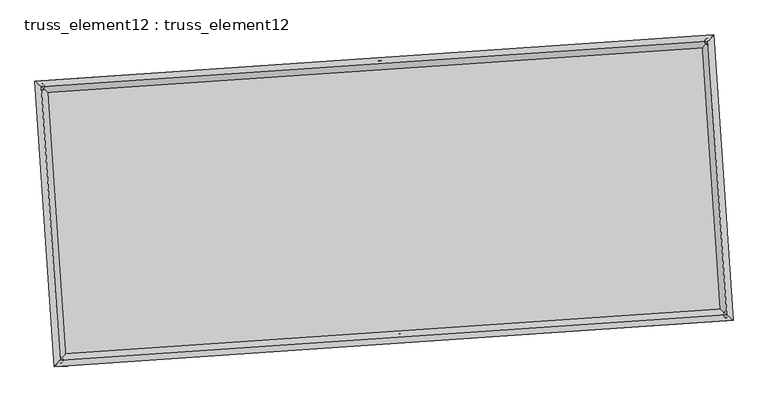
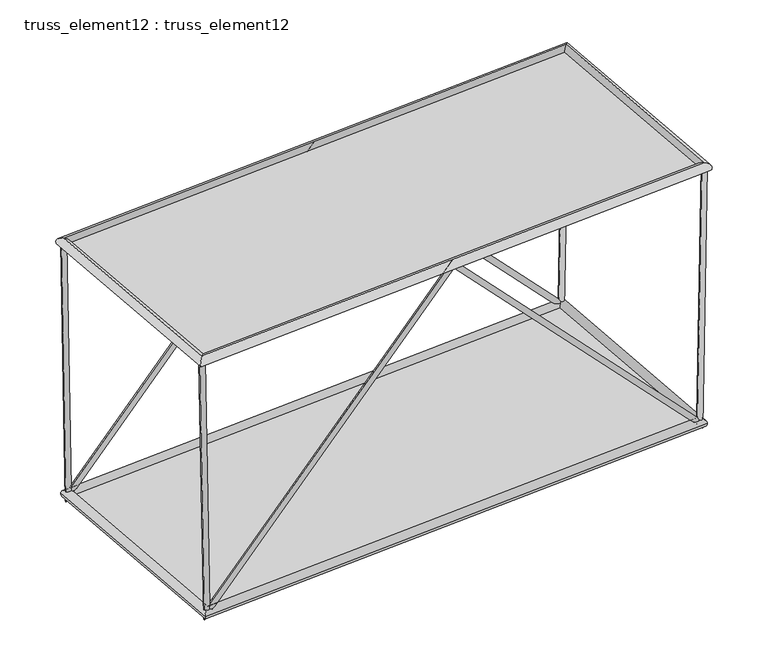
"""IFC4 building model written with IfcOpenShell, lengths in millimetres: plate geometry, truss_element12 : truss_element12."""

from ifc_helpers import new_model, si_unit, frame, origin, origin_with_axes, place, context, project, spatial, polyline, circle_curve, ellipse_curve, outline, extrude, source, transform, mapped, element, save
from ifc_brep_helpers import plane_surface, cylinder_surface, advanced_brep


def truss_element12_truss_element12_2665aa7a(model_context):
    return source(origin(), model_context, "Body", "SolidModel", [
        advanced_brep(
        [(-3754.7580634, 2270.0997186, 5000.0878443), (-3853.8452977, 2256.7395966, 4998.2914205), (-3667.1235212, 2276.0751849, 121.8973883), (-3761.8633617, 2263.0114952, -121.8973883), (1064.4357247, 2598.7022236, 5071.2944643), (1064.8732295, 2592.1283152, 4927.0589346), (5794.5966137, 2921.2339136, 121.8875614), (5890.1643633, 2921.1465749, -121.8875614), (5883.6190751, 2927.3040168, 5000.0761995), (5983.6021946, 2927.5177455, 4998.2513335)],
        [
            (0, 1, circle_curve(frame((-3804.3016806, 2263.4196576, 4999.1896324), z_axis=(-0.01796164783284105, -0.001224736487108711, 0.9998379264799201), x_axis=(-0.13360156854289684, 0.9910344161296608, -0.0011861405566435394)), 50.0)),
            (1, 0, circle_curve(frame((-3804.3016806, 2263.4196576, 4999.1896324), z_axis=(-0.01796164783284105, -0.001224736487108711, 0.9998379264799201), x_axis=(-0.13360156854289684, 0.9910344161296608, -0.0011861405566435394)), 50.0)),
            (0, 2),
            (2, 3, ellipse_curve(frame((-3714.4934414, 2269.54334, 0.0), z_axis=(-0.9290710914132946, -0.06334982599361827, 0.36443614892966897), x_axis=(0.36359189471660175, 0.024791949158535876, 0.9312283787306485)), 131.1845933, 50.0)),
            (3, 1),
            (3, 2, ellipse_curve(frame((-3714.4934414, 2269.54334, 0.0), z_axis=(-0.9290710914132946, -0.06334982599361827, 0.36443614892966897), x_axis=(0.36359189471660175, 0.024791949158535876, 0.9312283787306485)), 131.1845933, 50.0)),
            (2, 4),
            (4, 5, ellipse_curve(frame((1064.6544771, 2595.4152694, 4999.1766994), z_axis=(-0.9976833933192731, -0.06802823804080864, 7.432364115803836e-05), x_axis=(-7.415146271941529e-05, -5.056106363908644e-06, -0.9999999972379982)), 72.2747993, 50.0)),
            (5, 3),
            (5, 4, ellipse_curve(frame((1064.6544771, 2595.4152694, 4999.1766994), z_axis=(-0.9976833933192731, -0.06802823804080864, 7.432364115803836e-05), x_axis=(-7.415146271941529e-05, -5.056106363908644e-06, -0.9999999972379982)), 72.2747993, 50.0)),
            (4, 6),
            (6, 7, ellipse_curve(frame((5842.3804885, 2921.1902443, 0.0), z_axis=(-0.9291499210086431, -0.06335520108406349, -0.3642341867332474), x_axis=(-0.3633904003865968, -0.024778210026129826, 0.9313073913669803)), 131.1628889, 50.0)),
            (7, 5),
            (7, 6, ellipse_curve(frame((5842.3804885, 2921.1902443, 0.0), z_axis=(-0.9291499210086431, -0.06335520108406349, -0.3642341867332474), x_axis=(-0.3633904003865968, -0.024778210026129826, 0.9313073913669803)), 131.1628889, 50.0)),
            (8, 9, circle_curve(frame((5933.6106348, 2927.4108811, 4999.1637665), z_axis=(0.018246029263403518, 0.0012441273758179582, 0.999832753295866), x_axis=(-0.002159632777743711, 0.9999969420719114, -0.0012049203674651952)), 50.0)),
            (9, 8, circle_curve(frame((5933.6106348, 2927.4108811, 4999.1637665), z_axis=(0.018246029263403518, 0.0012441273758179582, 0.999832753295866), x_axis=(-0.002159632777743711, 0.9999969420719114, -0.0012049203674651952)), 50.0)),
            (6, 8),
            (9, 7),
        ],
        [
            plane_surface(frame((-3804.3016806, 2313.4196201, 4999.2508791), z_axis=(-0.01796164783284129, -0.0012247364871103106, 0.9998379264799201), x_axis=(0.9998386765909434, -2.2001834880214226e-05, 0.017961634357437358))),
            cylinder_surface(frame((-3804.3016806, 2263.4196576, 4999.1896324), z_axis=(-0.017961647832841054, -0.0012247364871087111, 0.9998379264799203), x_axis=(-0.13360156854289684, 0.9910344161296608, -0.0011861405566435394)), 50.0),
            cylinder_surface(frame((-3714.4934414, 2269.54334, 0.0), z_axis=(-0.6902549710503425, -0.04706586257112859, -0.7220338492901331), x_axis=(-0.02041985235552244, 0.9987518471124956, -0.04558264493375449)), 50.0),
            cylinder_surface(frame((1064.6544771, 2595.4152694, 4999.1766994), z_axis=(-0.6901478836925806, -0.047058560691284036, 0.7221366840843338), x_axis=(-0.11534776843769325, 0.9922790733696444, -0.04557557316287201)), 50.0),
            plane_surface(frame((5933.6106348, 2877.4109198, 4999.2259832), z_axis=(0.018246029263402925, 0.0012441273758166639, 0.999832753295866), x_axis=(0.9998335273514882, -2.270416412919475e-05, -0.01824601513760983))),
            cylinder_surface(frame((5842.3804885, 2921.1902443, 0.0), z_axis=(-0.018246029263403518, -0.0012441273758179582, -0.999832753295866), x_axis=(-0.002159632777743711, 0.9999969420719114, -0.0012049203674651952)), 50.0),
        ],
        [
            (0, [[1, 2]]),
            (1, [[-1, 3, 4, 5]]),
            (1, [[-2, -5, 6, -3]]),
            (2, [[-4, 7, 8, 9]]),
            (2, [[-6, -9, 10, -7]]),
            (3, [[-8, 11, 12, 13]]),
            (3, [[-10, -13, 14, -11]]),
            (4, [[15, 16]]),
            (5, [[-12, 17, -16, 18]]),
            (5, [[-14, -18, -15, -17]]),
        ],
    ),
        advanced_brep(
        [(-3482.6451105, -1720.6338657, 5000.0878443), (-3581.7323448, -1733.9939877, 4998.2914205), (-3395.0105682, -1714.6583994, 121.8973883), (-3489.7504088, -1727.7220891, -121.8973883), (1336.5486776, -1392.0313607, 5071.2944643), (1336.9861824, -1398.6052691, 4927.0589346), (6066.7095666, -1069.4996707, 121.8875614), (6162.2773162, -1069.5870094, -121.8875614), (6155.732028, -1063.4295675, 5000.0761995), (6255.7151475, -1063.2158388, 4998.2513335)],
        [
            (0, 1, circle_curve(frame((-3532.1887277, -1727.3139267, 4999.1896324), z_axis=(-0.0179616478328406, -0.001224736487108671, 0.9998379264799202), x_axis=(-0.1336015685428968, 0.9910344161296607, -0.0011861405566435178)), 50.0)),
            (1, 0, circle_curve(frame((-3532.1887277, -1727.3139267, 4999.1896324), z_axis=(-0.0179616478328406, -0.001224736487108671, 0.9998379264799202), x_axis=(-0.1336015685428968, 0.9910344161296607, -0.0011861405566435178)), 50.0)),
            (0, 2),
            (2, 3, ellipse_curve(frame((-3442.3804885, -1721.1902443, 0.0), z_axis=(-0.9290710914132937, -0.06334982599361812, 0.364436148929671), x_axis=(0.3635918947166038, 0.024791949158535984, 0.9312283787306476)), 131.1845933, 50.0)),
            (3, 1),
            (3, 2, ellipse_curve(frame((-3442.3804885, -1721.1902443, 0.0), z_axis=(-0.9290710914132937, -0.06334982599361812, 0.364436148929671), x_axis=(0.3635918947166038, 0.024791949158535984, 0.9312283787306476)), 131.1845933, 50.0)),
            (2, 4),
            (4, 5, ellipse_curve(frame((1336.76743, -1395.3183149, 4999.1766994), z_axis=(-0.997683393319273, -0.06802823804080865, 7.432364116132821e-05), x_axis=(-7.415146272295163e-05, -5.056106364052789e-06, -0.9999999972379982)), 72.2747993, 50.0)),
            (5, 3),
            (5, 4, ellipse_curve(frame((1336.76743, -1395.3183149, 4999.1766994), z_axis=(-0.997683393319273, -0.06802823804080865, 7.432364116132821e-05), x_axis=(-7.415146272295163e-05, -5.056106364052789e-06, -0.9999999972379982)), 72.2747993, 50.0)),
            (4, 6),
            (6, 7, ellipse_curve(frame((6114.4934414, -1069.54334, 0.0), z_axis=(-0.9291499210086436, -0.06335520108406373, -0.36423418673324576), x_axis=(-0.36339040038659537, -0.02477821002612974, 0.9313073913669809)), 131.1628889, 50.0)),
            (7, 5),
            (7, 6, ellipse_curve(frame((6114.4934414, -1069.54334, 0.0), z_axis=(-0.9291499210086436, -0.06335520108406373, -0.36423418673324576), x_axis=(-0.36339040038659537, -0.02477821002612974, 0.9313073913669809)), 131.1628889, 50.0)),
            (8, 9, circle_curve(frame((6205.7235877, -1063.3227032, 4999.1637665), z_axis=(0.01824602926340396, 0.0012441273758180466, 0.999832753295866), x_axis=(-0.0021596327777439264, 0.9999969420719114, -0.0012049203674652786)), 50.0)),
            (9, 8, circle_curve(frame((6205.7235877, -1063.3227032, 4999.1637665), z_axis=(0.01824602926340396, 0.0012441273758180466, 0.999832753295866), x_axis=(-0.0021596327777439264, 0.9999969420719114, -0.0012049203674652786)), 50.0)),
            (6, 8),
            (9, 7),
        ],
        [
            plane_surface(frame((-3532.1887277, -1677.3139642, 4999.2508791), z_axis=(-0.01796164783284129, -0.001224736487110304, 0.9998379264799201), x_axis=(0.9998386765909434, -2.2001834880214226e-05, 0.017961634357437358))),
            cylinder_surface(frame((-3532.1887277, -1727.3139267, 4999.1896324), z_axis=(-0.0179616478328406, -0.001224736487108671, 0.9998379264799202), x_axis=(-0.1336015685428968, 0.9910344161296607, -0.0011861405566435178)), 50.0),
            cylinder_surface(frame((-3442.3804885, -1721.1902443, 0.0), z_axis=(-0.6902549710503453, -0.04706586257112873, -0.7220338492901307), x_axis=(-0.02041985235552259, 0.9987518471124958, -0.04558264493375463)), 50.0),
            cylinder_surface(frame((1336.76743, -1395.3183149, 4999.1766994), z_axis=(-0.6901478836925787, -0.047058560691283995, 0.7221366840843358), x_axis=(-0.11534776843769351, 0.9922790733696444, -0.045575573162871884)), 50.0),
            plane_surface(frame((6205.7235877, -1113.3226645, 4999.2259832), z_axis=(0.018246029263402925, 0.0012441273758166589, 0.999832753295866), x_axis=(0.9998335273514882, -2.270416412875066e-05, -0.01824601513760983))),
            cylinder_surface(frame((6114.4934414, -1069.54334, 0.0), z_axis=(-0.01824602926340396, -0.0012441273758180466, -0.999832753295866), x_axis=(-0.0021596327777439264, 0.9999969420719114, -0.0012049203674652786)), 50.0),
        ],
        [
            (0, [[1, 2]]),
            (1, [[-1, 3, 4, 5]]),
            (1, [[-2, -5, 6, -3]]),
            (2, [[-4, 7, 8, 9]]),
            (2, [[-6, -9, 10, -7]]),
            (3, [[-8, 11, 12, 13]]),
            (3, [[-10, -13, 14, -11]]),
            (4, [[15, 16]]),
            (5, [[-12, 17, -16, 18]]),
            (5, [[-14, -18, -15, -17]]),
        ],
    ),
        advanced_brep(
        [(-3532.1954768, -1727.321407, 4909.1896327), (-3532.1819786, -1727.3064464, 5089.1896321), (-3804.2939786, 2263.4131627, 5089.1896321), (-3804.3093826, 2263.4261525, 4909.1896327), (5933.6043616, 2927.4034333, 5089.1637662), (5933.616908, 2927.418329, 4909.1637667), (6205.7163616, -1063.3161758, 5089.1637662), (6205.7308138, -1063.3292305, 4909.1637667)],
        [
            (0, 1, ellipse_curve(frame((-3532.1887277, -1727.3139267, 4999.1896324), z_axis=(-0.7535719234029808, 0.6573654662782497, 1.873871565689062e-06), x_axis=(-0.6573654662756035, -0.7535719234052891, 1.8738715718147376e-06)), 127.2792206, 90.0)),
            (1, 2),
            (2, 3, ellipse_curve(frame((-3804.3016806, 2263.4196576, 4999.1896324), z_axis=(-0.6573654662756034, -0.7535719234052891, 1.8738715680492458e-06), x_axis=(0.7535719234029807, -0.6573654662782497, -1.8738715619235709e-06)), 127.2792206, 90.0)),
            (3, 0),
            (1, 0, ellipse_curve(frame((-3532.1887277, -1727.3139267, 4999.1896324), z_axis=(-0.7535719234029808, 0.6573654662782497, 1.873871565689062e-06), x_axis=(-0.6573654662756035, -0.7535719234052891, 1.8738715718147376e-06)), 127.2792206, 90.0)),
            (3, 2, ellipse_curve(frame((-3804.3016806, 2263.4196576, 4999.1896324), z_axis=(-0.6573654662756034, -0.7535719234052891, 1.8738715680492458e-06), x_axis=(0.7535719234029807, -0.6573654662782497, -1.8738715619235709e-06)), 127.2792206, 90.0)),
            (2, 4),
            (4, 5, ellipse_curve(frame((5933.6106348, 2927.4108811, 4999.1637665), z_axis=(-0.7535719234029815, 0.6573654662782488, 1.8738715711120572e-06), x_axis=(-0.6573654662756028, -0.7535719234052898, 1.8738715588607595e-06)), 127.2792206, 90.0)),
            (5, 3),
            (5, 4, ellipse_curve(frame((5933.6106348, 2927.4108811, 4999.1637665), z_axis=(-0.7535719234029815, 0.6573654662782488, 1.8738715711120572e-06), x_axis=(-0.6573654662756028, -0.7535719234052898, 1.8738715588607595e-06)), 127.2792206, 90.0)),
            (4, 6),
            (6, 7, ellipse_curve(frame((6205.7235877, -1063.3227032, 4999.1637665), z_axis=(0.6573654662756028, 0.7535719234052897, -1.8738715626262506e-06), x_axis=(-0.7535719234029813, 0.6573654662782492, 1.8738715748775483e-06)), 127.2792206, 90.0)),
            (7, 5),
            (7, 6, ellipse_curve(frame((6205.7235877, -1063.3227032, 4999.1637665), z_axis=(0.6573654662756028, 0.7535719234052897, -1.8738715626262506e-06), x_axis=(-0.7535719234029813, 0.6573654662782492, 1.8738715748775483e-06)), 127.2792206, 90.0)),
            (6, 1),
            (0, 7),
        ],
        [
            cylinder_surface(frame((-3532.1887277, -1727.3139267, 4999.1896324), z_axis=(0.0680282382287005, -0.9976833960748768, 0.0), x_axis=(-0.9976833928446476, -0.06802823800844345, 8.04702389176603e-05)), 90.0),
            cylinder_surface(frame((-3804.3016806, 2263.4196576, 4999.1896324), z_axis=(-0.9976833960713734, -0.0680282382284634, 2.6500545813490755e-06), x_axis=(-0.06802823781696342, 0.99768339306793, 7.782018434000411e-05)), 90.0),
            cylinder_surface(frame((5933.6106348, 2927.4108811, 4999.1637665), z_axis=(-0.06802823822870241, 0.9976833960748765, 0.0), x_axis=(0.9976833932561474, 0.06802823803650399, 7.517012975801648e-05)), 90.0),
            cylinder_surface(frame((6205.7235877, -1063.3227032, 4999.1637665), z_axis=(0.9976833960713734, 0.06802823822846327, -2.6500545866742844e-06), x_axis=(0.06802823822846325, -0.9976833930398714, 7.782018432800353e-05)), 90.0),
        ],
        [
            (0, [[1, 2, 3, 4]]),
            (0, [[5, -4, 6, -2]]),
            (1, [[-3, 7, 8, 9]]),
            (1, [[-6, -9, 10, -7]]),
            (2, [[-8, 11, 12, 13]]),
            (2, [[-10, -13, 14, -11]]),
            (3, [[-12, 15, -1, 16]]),
            (3, [[-14, -16, -5, -15]]),
        ],
    ),
        advanced_brep(
        [(-3358.7115243, -1625.2761972, 0.0), (-3526.0494527, -1817.1042913, 0.0), (-3810.4074885, 2353.2123043, 0.0), (-3618.5793943, 2185.8743758, 0.0), (5926.0494527, 3017.1042913, 0.0), (5758.7115243, 2825.2761972, 0.0), (6210.4074885, -1153.2123043, 0.0), (6018.5793943, -985.8743758, 0.0)],
        [
            (0, 1, ellipse_curve(frame((-3442.3804885, -1721.1902443, 0.0), z_axis=(-0.7535719234054581, 0.6573654662780807, 0.0), x_axis=(-0.6573654662780806, -0.7535719234054581, 0.0)), 127.2792206, 90.0)),
            (1, 2),
            (2, 3, ellipse_curve(frame((-3714.4934414, 2269.54334, 0.0), z_axis=(-0.6573654662780806, -0.7535719234054581, 0.0), x_axis=(0.753571923405458, -0.6573654662780808, 0.0)), 127.2792206, 90.0)),
            (3, 0),
            (1, 0, ellipse_curve(frame((-3442.3804885, -1721.1902443, 0.0), z_axis=(-0.7535719234054581, 0.6573654662780807, 0.0), x_axis=(-0.6573654662780806, -0.7535719234054581, 0.0)), 127.2792206, 90.0)),
            (3, 2, ellipse_curve(frame((-3714.4934414, 2269.54334, 0.0), z_axis=(-0.6573654662780806, -0.7535719234054581, 0.0), x_axis=(0.753571923405458, -0.6573654662780808, 0.0)), 127.2792206, 90.0)),
            (2, 4),
            (4, 5, ellipse_curve(frame((5842.3804885, 2921.1902443, 0.0), z_axis=(-0.7535719234054589, 0.6573654662780797, 0.0), x_axis=(-0.6573654662780798, -0.7535719234054589, 0.0)), 127.2792206, 90.0)),
            (5, 3),
            (5, 4, ellipse_curve(frame((5842.3804885, 2921.1902443, 0.0), z_axis=(-0.7535719234054589, 0.6573654662780797, 0.0), x_axis=(-0.6573654662780798, -0.7535719234054589, 0.0)), 127.2792206, 90.0)),
            (4, 6),
            (6, 7, ellipse_curve(frame((6114.4934414, -1069.54334, 0.0), z_axis=(0.6573654662780798, 0.7535719234054588, 0.0), x_axis=(-0.7535719234054589, 0.6573654662780799, 0.0)), 127.2792206, 90.0)),
            (7, 5),
            (7, 6, ellipse_curve(frame((6114.4934414, -1069.54334, 0.0), z_axis=(0.6573654662780798, 0.7535719234054588, 0.0), x_axis=(-0.7535719234054589, 0.6573654662780799, 0.0)), 127.2792206, 90.0)),
            (6, 1),
            (0, 7),
        ],
        [
            cylinder_surface(frame((-3442.3804885, -1721.1902443, 0.0), z_axis=(0.06802823822870041, -0.9976833960748767, 0.0), x_axis=(-0.9976833960748767, -0.06802823822870041, 0.0)), 90.0),
            cylinder_surface(frame((-3714.4934414, 2269.54334, 0.0), z_axis=(-0.9976833960748765, -0.06802823822870256, 0.0), x_axis=(-0.06802823822870256, 0.9976833960748765, 0.0)), 90.0),
            cylinder_surface(frame((5842.3804885, 2921.1902443, 0.0), z_axis=(-0.06802823822870269, 0.9976833960748765, 0.0), x_axis=(0.9976833960748765, 0.06802823822870269, 0.0)), 90.0),
            cylinder_surface(frame((6114.4934414, -1069.54334, 0.0), z_axis=(0.9976833960748765, 0.06802823822870234, 0.0), x_axis=(0.06802823822870234, -0.9976833960748765, 0.0)), 90.0),
        ],
        [
            (0, [[1, 2, 3, 4]]),
            (0, [[5, -4, 6, -2]]),
            (1, [[-3, 7, 8, 9]]),
            (1, [[-6, -9, 10, -7]]),
            (2, [[-8, 11, 12, 13]]),
            (2, [[-10, -13, 14, -11]]),
            (3, [[-12, 15, -1, 16]]),
            (3, [[-14, -16, -5, -15]]),
        ],
    ),
        extrude(outline(polyline([(-3442.3804885, -1721.1902443), (-3714.4934414, 2269.54334), (5842.3804885, 2921.1902443), (6114.4934414, -1069.54334), (-3442.3804885, -1721.1902443)])), origin_with_axes(), (0.0, 0.0, 1.0), 20.0),
        extrude(outline(polyline([(-2000.0, 4880.2617914), (2000.0, 4880.2617914), (2000.0, -4880.2617913), (-2000.0, -4880.2617913), (-2000.0, 4880.2617914)])), frame((1200.7109536, 600.0484772, 4999.1766994), z_axis=(2.643915454209429e-06, 1.8027854870050657e-07, 0.9999999999964887), x_axis=(-0.06802823822870088, 0.9976833960748767, 0.0)), (0.0, 0.0, 1.0), 20.0),
    ])


if __name__ == "__main__":
    model = new_model("IFC4")
    model_context = context("Model", 3, world=origin())
    ifc_project = project(units=[si_unit("LENGTHUNIT", "METRE", prefix="MILLI")], contexts=[model_context])
    site = spatial("IfcSite", under=ifc_project)
    building = spatial("IfcBuilding", under=site)
    placement = place(None, origin())
    truss_element12_truss_element12_shape = truss_element12_truss_element12_2665aa7a(model_context)
    element("IfcPlate", 1, ObjectType="truss_element12 : truss_element12", at=placement, inside=building, context=model_context, shape_type="MappedRepresentation", body=[
        mapped(truss_element12_truss_element12_shape, transform((0.0, 0.0, 0.0), x_axis=(1.0, 0.0, 0.0), y_axis=(0.0, 1.0, 0.0), z_axis=(0.0, 0.0, 1.0))),
    ])
    save(model, "model.ifc")

# Revit data of these elements
# Type "truss_element12 : truss_element12"
#   steellbar1 = 90 mm
#   steelbar2 = 50 mm
#   offset1 = 5000 mm
#   M = Default Roof
# Element 1 (IfcPlate, "truss_element12 : truss_element12")
#   Materials on its faces: "Default Roof"
# Materials
#   "Default Roof": class "Miscellaneous", colour RGB 0 127 0, transparency 0, Comments = "Rendering appearance not upgraded Rendering appearance not upgraded ", Cost = 0
